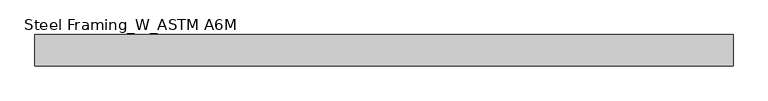
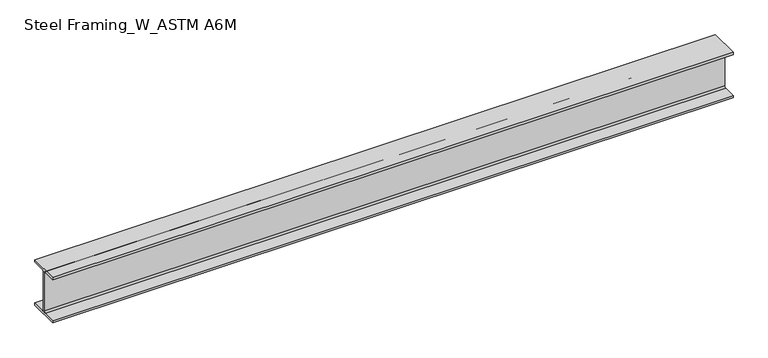
"""IFC4 building model written with IfcOpenShell, lengths in millimetres: beam geometry, Steel Framing_W_ASTM A6M : H_SB_AR_S02_W200x31.3_B6."""

import ifcopenshell
import ifcopenshell.guid

model = None  # the IFC model being written
_history = None  # IfcOwnerHistory: only IFC2X3 demands one
_inside = {}  # id of a spatial element -> (the spatial element, [elements in it])
_under = {}  # id of a project, library or spatial element -> (it, [spatial elements below it])
_declared = {}  # id of a project -> (the project, [libraries it declares])
_typed = {}  # id of a type object -> (the type object, [elements of that type])
_made_of = {}  # id of a material, layer set ... -> (it, [elements and type objects made of it])


def new_model(schema):
    """Start an empty IFC model of exactly this schema.

    Asked for "IFC4X3", IfcOpenShell would pick the latest addendum, in which some entities
    have other attributes; the version numbers below select the first issue.
    IFC2X3 requires an IfcOwnerHistory on every rooted entity: one is made here for all.
    """
    global model, _history
    if schema == "IFC4X3":
        model = ifcopenshell.file(schema_version=(4, 3, 0, 0))
    else:
        model = ifcopenshell.file(schema=schema)
    _inside.clear()
    _under.clear()
    _declared.clear()
    _typed.clear()
    _made_of.clear()
    _history = None
    if model.schema == "IFC2X3":
        org = make("IfcOrganization", Name="unknown")
        user = make(
            "IfcPersonAndOrganization",
            ThePerson=make("IfcPerson", FamilyName="unknown"),
            TheOrganization=org,
        )
        app = make(
            "IfcApplication",
            ApplicationDeveloper=org,
            Version="unknown",
            ApplicationFullName="unknown",
            ApplicationIdentifier="unknown",
        )
        _history = make(
            "IfcOwnerHistory",
            OwningUser=user,
            OwningApplication=app,
            ChangeAction="ADDED",
            CreationDate=0,
        )
    return model


def make(cls, **values):
    """One entity of the class cls with the attributes given. An attribute that is None is left unset."""
    return model.create_entity(
        cls, **{name: value for name, value in values.items() if value is not None}
    )


def rooted(cls, **values):
    """An entity with a GlobalId (a new one), such as an element, a storey or a relation."""
    return make(cls, GlobalId=ifcopenshell.guid.new(), OwnerHistory=_history, **values)


def si_unit(unit_type, name, prefix=None):
    """IfcSIUnit, for example si_unit("LENGTHUNIT", "METRE", prefix="MILLI")."""
    return make("IfcSIUnit", UnitType=unit_type, Prefix=prefix, Name=name)


def assignment(units):
    """IfcUnitAssignment: the units of a project."""
    return None if units is None else make("IfcUnitAssignment", Units=units)


def point(xyz):
    """IfcCartesianPoint."""
    return None if xyz is None else make("IfcCartesianPoint", Coordinates=xyz)


def direction(xyz):
    """IfcDirection."""
    return None if xyz is None else make("IfcDirection", DirectionRatios=xyz)


def frame(location, z_axis=None, x_axis=None):
    """IfcAxis2Placement3D, a coordinate frame: its origin and axes. An axis left out is left unset."""
    return make(
        "IfcAxis2Placement3D",
        Location=point(location),
        Axis=direction(z_axis),
        RefDirection=direction(x_axis),
    )


def frame_2d(location, x_axis=None):
    """IfcAxis2Placement2D, a coordinate frame in the plane: its origin and x axis."""
    return make(
        "IfcAxis2Placement2D", Location=point(location), RefDirection=direction(x_axis)
    )


def origin():
    """The frame at (0, 0, 0) with its axes left unset."""
    return frame((0.0, 0.0, 0.0))


def place(relative_to, where):
    """IfcLocalPlacement: puts the frame where relative to a parent placement (None: the world)."""
    return make(
        "IfcLocalPlacement", PlacementRelTo=relative_to, RelativePlacement=where
    )


def context(
    kind, dimensions, precision=None, world=None, true_north=None, identifier=None
):
    """IfcGeometricRepresentationContext, for example the 3D "Model" context."""
    return make(
        "IfcGeometricRepresentationContext",
        ContextIdentifier=identifier,
        ContextType=kind,
        CoordinateSpaceDimension=dimensions,
        Precision=precision,
        WorldCoordinateSystem=world,
        TrueNorth=true_north,
    )


def project(units=None, contexts=None):
    """IfcProject with its units and contexts."""
    return rooted(
        "IfcProject",
        Name="project",
        RepresentationContexts=contexts,
        UnitsInContext=assignment(units),
    )


def spatial(cls, under=None, at=None, **own):
    """A site, building, storey or space (cls), placed at a placement, below another one or the project."""
    s = rooted(cls, ObjectPlacement=at, **own)
    if under is not None:
        _under.setdefault(under.id(), (under, []))[1].append(s)
    return s


def polyline(points):
    """IfcPolyline through the points."""
    return make("IfcPolyline", Points=[point(p) for p in points])


def circle_curve(where, radius):
    """IfcCircle in the frame where."""
    return make("IfcCircle", Position=where, Radius=radius)


def trimmed(basis, trim1, trim2, sense, master):
    """IfcTrimmedCurve: the piece of a basis curve between two trims."""
    return make(
        "IfcTrimmedCurve",
        BasisCurve=basis,
        Trim1=trim1,
        Trim2=trim2,
        SenseAgreement=sense,
        MasterRepresentation=master,
    )


def segment(curve, same_sense, transition):
    """IfcCompositeCurveSegment."""
    return make(
        "IfcCompositeCurveSegment",
        Transition=transition,
        SameSense=same_sense,
        ParentCurve=curve,
    )


def composite_curve(segments, self_intersect=None):
    """IfcCompositeCurve: segments joined end to end."""
    return make("IfcCompositeCurve", Segments=segments, SelfIntersect=self_intersect)


def outline(outer, holes=None, kind="AREA"):
    """IfcArbitraryClosedProfileDef: a profile drawn as a closed curve; with holes, ...WithVoids."""
    if holes is None:
        return make("IfcArbitraryClosedProfileDef", ProfileType=kind, OuterCurve=outer)
    return make(
        "IfcArbitraryProfileDefWithVoids",
        ProfileType=kind,
        OuterCurve=outer,
        InnerCurves=holes,
    )


def extrude(swept, where, along, depth):
    """IfcExtrudedAreaSolid: the profile swept, set in the frame where, extruded along a direction by depth."""
    return make(
        "IfcExtrudedAreaSolid",
        SweptArea=swept,
        Position=where,
        ExtrudedDirection=direction(along),
        Depth=depth,
    )


def shape(context_of_items, identifier, shape_type, items):
    """IfcShapeRepresentation: the items that make up one representation, for example the "Body"."""
    return make(
        "IfcShapeRepresentation",
        ContextOfItems=context_of_items,
        RepresentationIdentifier=identifier,
        RepresentationType=shape_type,
        Items=items,
    )


def source(mapping_origin, context_of_items, identifier, shape_type, items):
    """IfcRepresentationMap: a shape defined once, which mapped items show again and again."""
    return make(
        "IfcRepresentationMap",
        MappingOrigin=mapping_origin,
        MappedRepresentation=shape(context_of_items, identifier, shape_type, items),
    )


def transform(
    local_origin,
    x_axis=None,
    y_axis=None,
    z_axis=None,
    scale=None,
    scale2=None,
    scale3=None,
    uniform=True,
):
    """IfcCartesianTransformationOperator3D, or its non-uniform kind. x_axis, y_axis, z_axis: its Axis1, 2, 3."""
    if uniform:
        return make(
            "IfcCartesianTransformationOperator3D",
            Axis1=direction(x_axis),
            Axis2=direction(y_axis),
            LocalOrigin=point(local_origin),
            Scale=scale,
            Axis3=direction(z_axis),
        )
    return make(
        "IfcCartesianTransformationOperator3DnonUniform",
        Axis1=direction(x_axis),
        Axis2=direction(y_axis),
        LocalOrigin=point(local_origin),
        Scale=scale,
        Axis3=direction(z_axis),
        Scale2=scale2,
        Scale3=scale3,
    )


def mapped(mapping_source, mapping_target):
    """IfcMappedItem: shows the shape of a source again, moved by a transform."""
    return make(
        "IfcMappedItem", MappingSource=mapping_source, MappingTarget=mapping_target
    )


def made_of(thing, what):
    """Note that an element or type object is made of a material, layer set ...; save() writes the relation."""
    if what is not None:
        _made_of.setdefault(what.id(), (what, []))[1].append(thing)
    return thing


def element(
    cls,
    number,
    at=None,
    inside=None,
    cuts=None,
    type_object=None,
    material=None,
    context=None,
    identifier="Body",
    shape_type=None,
    held_by="IfcProductDefinitionShape",
    body=None,
    shapes=None,
    **own,
):
    """One element of the class cls, such as IfcWall. Its Tag is "e" and its number.

    at: its placement. inside: the storey or other place that contains it. cuts: it is an
    opening in that element (IfcRelVoidsElement). A single representation is given by context,
    identifier, shape_type and body (its items); several are given by shapes. held_by: the class
    of the entity that holds the representations. save() writes the other relations.
    """
    e = rooted(cls, Tag="e%d" % number, ObjectPlacement=at, **own)
    if body is not None:
        shapes = [shape(context, identifier, shape_type, body)]
    if shapes is not None:
        e.Representation = make(held_by, Representations=shapes)
    if inside is not None:
        _inside.setdefault(inside.id(), (inside, []))[1].append(e)
    if cuts is not None:
        rooted(
            "IfcRelVoidsElement", RelatingBuildingElement=cuts, RelatedOpeningElement=e
        )
    if type_object is not None:
        _typed.setdefault(type_object.id(), (type_object, []))[1].append(e)
    return made_of(e, material)


def aggregate(whole, parts):
    """IfcRelAggregates: a whole, such as a stair, and the parts it consists of."""
    return rooted("IfcRelAggregates", RelatingObject=whole, RelatedObjects=parts)


def save(model, path):
    """Write the relations noted so far, then the file.

    IfcRelAggregates (storeys below a building ...), IfcRelContainedInSpatialStructure (elements
    in a storey), IfcRelDefinesByType, IfcRelAssociatesMaterial and IfcRelDeclares: one each for
    every whole, place, type object, material and project.
    """
    for whole, parts in _under.values():
        aggregate(whole, parts)
    for where, things in _inside.values():
        rooted(
            "IfcRelContainedInSpatialStructure",
            RelatedElements=things,
            RelatingStructure=where,
        )
    for kind, things in _typed.values():
        rooted("IfcRelDefinesByType", RelatedObjects=things, RelatingType=kind)
    for what, things in _made_of.values():
        rooted("IfcRelAssociatesMaterial", RelatedObjects=things, RelatingMaterial=what)
    for by, libraries in _declared.values():
        rooted("IfcRelDeclares", RelatingContext=by, RelatedDefinitions=libraries)
    model.write(path)


def steel_framing_w_astm_a6m_95b0337f(model_context):
    return source(origin(), model_context, "Body", "SweptSolid", [
        extrude(outline(composite_curve([segment(polyline([(67.0, -94.8), (67.0, -105.0), (-67.0, -105.0), (-67.0, -94.8), (-10.775, -94.8)]), True, "CONTINUOUS"), segment(trimmed(circle_curve(frame_2d((-10.775, -87.2)), 7.6), [point((-10.775, -94.8))], [point((-3.175, -87.2))], True, "CARTESIAN"), True, "CONTINUOUS"), segment(polyline([(-3.175, -87.2), (-3.175, 87.2)]), True, "CONTINUOUS"), segment(trimmed(circle_curve(frame_2d((-10.775, 87.2)), 7.6), [point((-3.175, 87.2))], [point((-10.775, 94.8))], True, "CARTESIAN"), True, "CONTINUOUS"), segment(polyline([(-10.775, 94.8), (-67.0, 94.8), (-67.0, 105.0), (67.0, 105.0), (67.0, 94.8), (10.775, 94.8)]), True, "CONTINUOUS"), segment(trimmed(circle_curve(frame_2d((10.775, 87.2)), 7.6), [point((10.775, 94.8))], [point((3.175, 87.2))], True, "CARTESIAN"), True, "CONTINUOUS"), segment(polyline([(3.175, 87.2), (3.175, -87.2)]), True, "CONTINUOUS"), segment(trimmed(circle_curve(frame_2d((10.775, -87.2)), 7.6), [point((3.175, -87.2))], [point((10.775, -94.8))], True, "CARTESIAN"), True, "CONTINUOUS"), segment(polyline([(10.775, -94.8), (67.0, -94.8)]), True, "CONTINUOUS")], self_intersect=False)), frame((-1487.2, 0.0, 0.0), z_axis=(1.0, 0.0, 0.0), x_axis=(0.0, 1.0, 0.0)), (0.0, 0.0, 1.0), 2974.4),
    ])


if __name__ == "__main__":
    model = new_model("IFC4")
    model_context = context("Model", 3, world=origin())
    ifc_project = project(units=[si_unit("LENGTHUNIT", "METRE", prefix="MILLI")], contexts=[model_context])
    site = spatial("IfcSite", under=ifc_project)
    building = spatial("IfcBuilding", under=site)
    placement = place(None, origin())
    steel_framing_w_astm_a6m_shape = steel_framing_w_astm_a6m_95b0337f(model_context)
    element("IfcBeam", 1, ObjectType="Steel Framing_W_ASTM A6M : H_SB_AR_S02_W200x31.3_B6", at=placement, inside=building, context=model_context, shape_type="MappedRepresentation", body=[
        mapped(steel_framing_w_astm_a6m_shape, transform((0.0, 0.0, 0.0), x_axis=(1.0, 0.0, 0.0), y_axis=(0.0, 1.0, 0.0), z_axis=(0.0, 0.0, 1.0))),
    ])
    save(model, "model.ifc")

# Revit data of these elements
# Type "Steel Framing_W_ASTM A6M : H_SB_AR_S02_W200x31.3_B6"
#   Type Mark = "B6"
#   Section Name Key = "W8x21"
#   Width = 13.4 cm
#   Web Thickness = 0.635 cm
#   Web Fillet = 0.76 cm
#   Warping Constant = 40800.0 cm⁶
#   Torsional Moment of Inertia = 11.70 cm⁴
#   Section Area = 39.7 cm²
#   Plastic Modulus weak axis = 93.2 cm³
#   Plastic Modulus strong axis = 334.0 cm³
#   Perimeter = 0.93 m²/m
#   Nominal Weight = 31.30 kgf/m
#   Moment of Inertia weak axis = 407.00 cm⁴
#   Moment of Inertia strong axis = 3130.00 cm⁴
#   Height = 21.0 cm
#   Flange Thickness = 1.02 cm
#   Elastic Modulus weak axis = 60.8 cm³
#   Elastic Modulus strong axis = 298.0 cm³
#   Centroid Vertical = 10.5 cm
#   Centroid Horizontal = 6.7 cm
#   Length [instance default] = 1500 mm
#   Structural Material [instance default] = Steel, 45-345
#   Bolt Spacing = 0
#   Assembly Code = ""
# Element 1 (IfcBeam, "Steel Framing_W_ASTM A6M : H_SB_AR_S02_W200x31.3_B6")
#   Materials on its faces: "Steel, 45-345"
# Materials
#   "Steel, 45-345": class "Metal", colour RGB 189 187 185, transparency 0, Description = "Steel 345 MPa", Cost = 0
